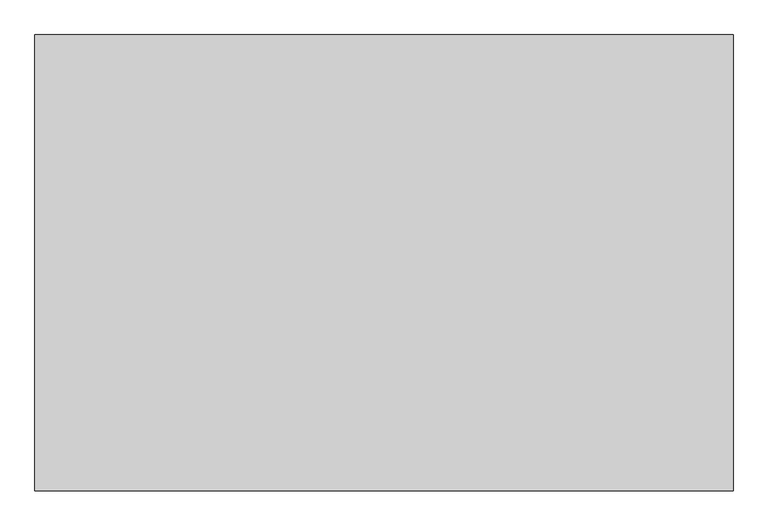
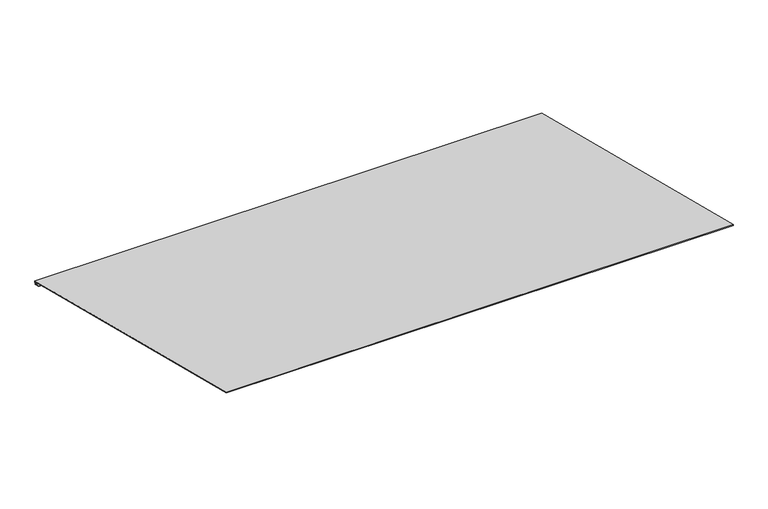
"""IFC4 building model written with IfcOpenShell, lengths in millimetres: proxy geometry, Gutter @ Roof001 : Gutter @ Roof001."""

from ifc_helpers import new_model, si_unit, frame, origin, place, context, project, spatial, polyline, outline, extrude, source, transform, mapped, element, save


def generic_models_4c0e396c(model_context):
    return source(origin(), model_context, "Body", "SweptSolid", [
        extrude(outline(polyline([(3064.132137, 41849.8246764), (4371.4558626, 41522.9928253), (4368.0267643, 41509.2764322), (4346.0295733, 41514.9618766), (4346.6651806, 41517.4210642), (4366.183559, 41512.3762993), (4368.3756601, 41521.1447038), (3064.132137, 41847.2055846), (3064.132137, 41849.8246764)])), frame((255.0171875, 0.0, 0.0), z_axis=(1.0, 0.0, 0.0), x_axis=(0.0, 1.0, 0.0)), (0.0, 0.0, 1.0), 1999.85),
    ])


if __name__ == "__main__":
    model = new_model("IFC4")
    model_context = context("Model", 3, world=origin())
    ifc_project = project(units=[si_unit("LENGTHUNIT", "METRE", prefix="MILLI")], contexts=[model_context])
    site = spatial("IfcSite", under=ifc_project)
    building = spatial("IfcBuilding", under=site)
    placement = place(None, origin())
    generic_models_shape = generic_models_4c0e396c(model_context)
    element("IfcBuildingElementProxy", 1, Name="Gutter @ Roof001 : Gutter @ Roof001", ObjectType="Gutter @ Roof001 : Gutter @ Roof001", at=placement, inside=building, context=model_context, shape_type="MappedRepresentation", body=[
        mapped(generic_models_shape, transform((0.0, 0.0, 0.0), x_axis=(1.0, 0.0, 0.0), y_axis=(0.0, 1.0, 0.0), z_axis=(0.0, 0.0, 1.0))),
    ])
    save(model, "model.ifc")

# Revit data of these elements
# Type "Gutter @ Roof001 : Gutter @ Roof001"
#   NameOverride = "Gutter @ Roof001"
# Element 1 (IfcBuildingElementProxy, "Gutter @ Roof001 : Gutter @ Roof001")
#   Materials on its faces: "CONT. SEAMLESS 16 GA COPPER BRAKE METAL GUTTER"
# Materials
#   "CONT. SEAMLESS 16 GA COPPER BRAKE METAL GUTTER": class "Unassigned", colour RGB 128 128 128, transparency 0
